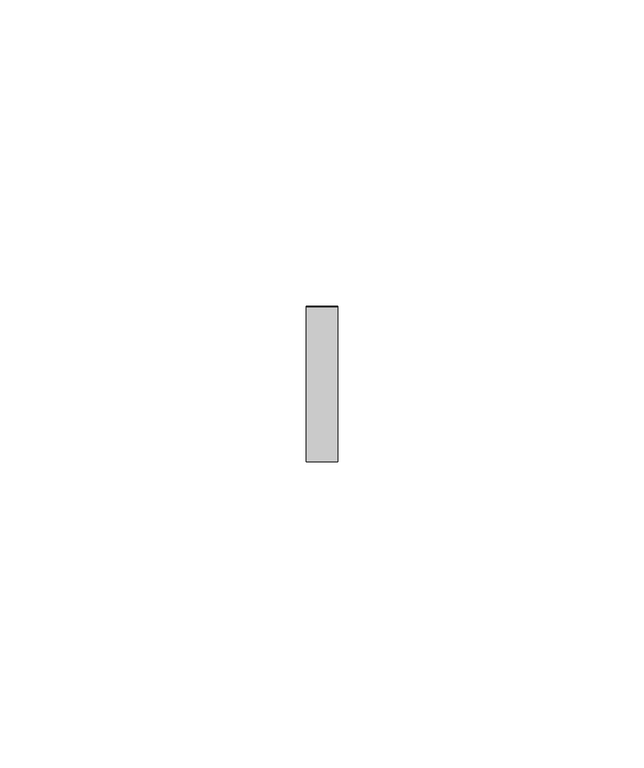
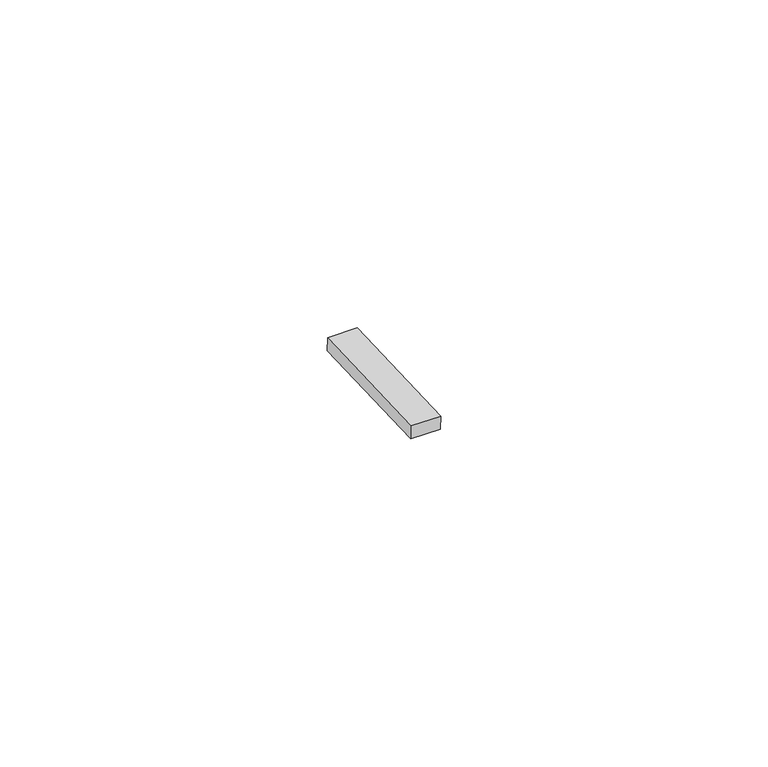
"""IFC4 building model written with IfcOpenShell, lengths in millimetres: proxy geometry, Inner panel:Inner panel:1:Inner panel:1 : Inner panel:Inner panel:300324:2:Inner panel:1:Inner panel:1 : Inner panel:Inner panel:300324:2 : Inner panel:Inner panel:1:Inner panel:1 : Inner panel:Inner panel:300324:300043:116 : Inner panel:Inner panel:1:Inner panel:1 : Inner panel:Inner panel:300324:2:Inner panel:1:Inner panel:1 : Inner panel:Inner panel:300324:2 : Inner panel:Inner panel:1:Inner panel:1 : Inner panel:Inner panel:300324:300043:308120."""

from ifc_helpers import new_model, si_unit, frame, origin, place, context, project, spatial, polyline, outline, extrude, source, transform, mapped, element, save


def generic_models_e1b1f6bb(model_context):
    return source(origin(), model_context, "Body", "SweptSolid", [
        extrude(outline(polyline([(0.0, -25.3999999), (0.0, 0.0), (5.2138089, 0.0), (5.2138089, -25.3999999), (0.0, -25.3999999)])), frame((593936.595117, -568123.7593241, 8806.3160403), z_axis=(0.0, -0.041630544712223896, 0.9991330730923502), x_axis=(-1.0, 0.0, 0.0)), (0.0, 0.0, 1.0), 2.4763745),
    ])


if __name__ == "__main__":
    model = new_model("IFC4")
    model_context = context("Model", 3, world=origin())
    ifc_project = project(units=[si_unit("LENGTHUNIT", "METRE", prefix="MILLI")], contexts=[model_context])
    site = spatial("IfcSite", under=ifc_project)
    building = spatial("IfcBuilding", under=site)
    placement = place(None, origin())
    generic_models_shape = generic_models_e1b1f6bb(model_context)
    element("IfcBuildingElementProxy", 1, Name="Inner panel:Inner panel:1:Inner panel:1 : Inner panel:Inner panel:300324:2:Inner panel:1:Inner panel:1 : Inner panel:Inner panel:300324:2 : Inner panel:Inner panel:1:Inner panel:1 : Inner panel:Inner panel:300324:300043:116 : Inner panel:Inner panel:1:Inner panel:1 : Inner panel:Inner panel:300324:2:Inner panel:1:Inner panel:1 : Inner panel:Inner panel:300324:2 : Inner panel:Inner panel:1:Inner panel:1 : Inner panel:Inner panel:300324:300043:308120", ObjectType="Inner panel:Inner panel:1:Inner panel:1 : Inner panel:Inner panel:300324:2:Inner panel:1:Inner panel:1 : Inner panel:Inner panel:300324:2 : Inner panel:Inner panel:1:Inner panel:1 : Inner panel:Inner panel:300324:300043:116 : Inner panel:Inner panel:1:Inner panel:1 : Inner panel:Inner panel:300324:2:Inner panel:1:Inner panel:1 : Inner panel:Inner panel:300324:2 : Inner panel:Inner panel:1:Inner panel:1 : Inner panel:Inner panel:300324:300043:308120", at=placement, inside=building, context=model_context, shape_type="MappedRepresentation", body=[
        mapped(generic_models_shape, transform((0.0, 0.0, 0.0), x_axis=(1.0, 0.0, 0.0), y_axis=(0.0, 1.0, 0.0), z_axis=(0.0, 0.0, 1.0))),
    ])
    save(model, "model.ifc")

# Revit data of these elements
# Type "Inner panel:Inner panel:1:Inner panel:1 : Inner panel:Inner panel:300324:2:Inner panel:1:Inner panel:1 : Inner panel:Inner panel:300324:2 : Inner panel:Inner panel:1:Inner panel:1 : Inner panel:Inner panel:300324:300043:116 : Inner panel:Inner panel:1:Inner panel:1 : Inner panel:Inner panel:300324:2:Inner panel:1:Inner panel:1 : Inner panel:Inner panel:300324:2 : Inner panel:Inner panel:1:Inner panel:1 : Inner panel:Inner panel:300324:300043:308120"
#   NameOverride = "Inner panel:Inner panel:1:Inner panel:1 : Inner panel:Inner panel:300324:2:Inner panel:1:Inner panel:1 : Inner panel:Inner panel:300324:2 : Inner panel:Inner panel:1:Inner panel:1 : Inner panel:Inner panel:300324:300043:308120"
#   ObjectTypeOverride = "Inner panel:1:Inner panel:1 : Inner panel:Inner panel:300324:2 : Inner panel:Inner panel:1:Inner panel:1 : Inner panel:Inner panel:300324:300043"
#   Reference = "Inner panel"
#   Tag = "308120"
# Element 1 (IfcBuildingElementProxy, "Inner panel:Inner panel:1:Inner panel:1 : Inner panel:Inner panel:300324:2:Inner panel:1:Inner panel:1 : Inner panel:Inner panel:300324:2 : Inner panel:Inner panel:1:Inner panel:1 : Inner panel:Inner panel:300324:300043:116 : Inner panel:Inner panel:1:Inner panel:1 : Inner panel:Inner panel:300324:2:Inner panel:1:Inner panel:1 : Inner panel:Inner panel:300324:2 : Inner panel:Inner panel:1:Inner panel:1 : Inner panel:Inner panel:300324:300043:308120")
#   Materials on its faces: "AT CLIP - 1\" WIDE NON ABSORBENT, WEATHER-RESISTANT NEOPRENE/EPDM/SBR FOAM"
# Materials
#   "AT CLIP - 1\" WIDE NON ABSORBENT, WEATHER-RESISTANT NEOPRENE/EPDM/SBR FOAM": class "Generic", colour RGB 85 85 85, transparency 0, Cost = 0
